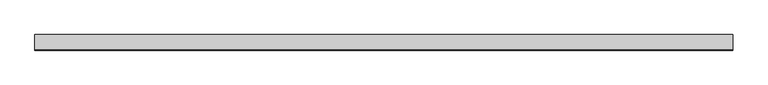
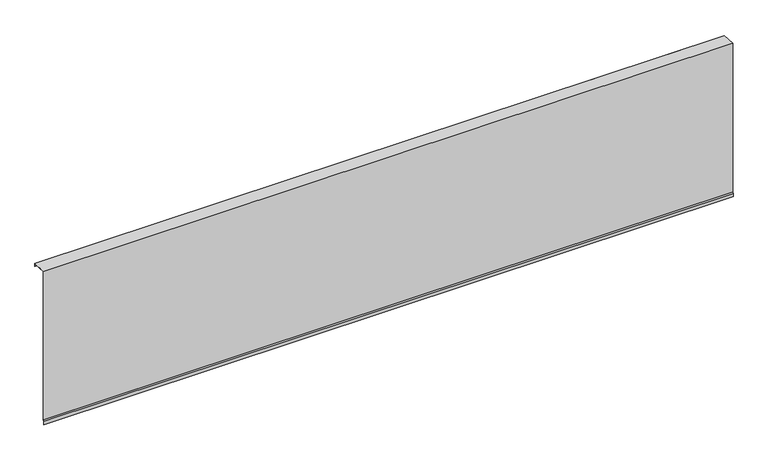
"""IFC4 building model written with IfcOpenShell, lengths in millimetres: proxy geometry, Generic Models 7:Generic Models 1:5:Generic Models 1:5 : Generic Models 7:Generic Models 1:337419:32 : Generic Models 7:Generic Models 1:5:Generic Models 1:5 : Generic Models 7:Generic Models 1:337419:311462."""

from ifc_helpers import new_model, si_unit, frame, origin, place, context, project, spatial, polyline, outline, extrude, source, transform, mapped, element, save


def generic_models_75d0ed6d(model_context):
    return source(origin(), model_context, "Body", "SweptSolid", [
        extrude(outline(polyline([(-579014.1851341, 3795.8885169), (-579025.7575229, 3779.361433), (-579025.7575229, 3725.3283058), (-579027.3450229, 3725.3283058), (-579027.3450229, 3779.8619698), (-579015.7726341, 3796.3890538), (-579015.7726341, 6180.6116872), (-578793.4990368, 6168.9628216), (-578793.4990368, 6125.115987), (-578795.0865368, 6125.115987), (-578795.0865368, 6167.4563403), (-579014.1851341, 6178.9388113), (-579014.1851341, 3795.8885169)])), frame((793360.8632437, 0.0, 0.0), z_axis=(1.0, 0.0, 0.0), x_axis=(0.0, 1.0, 0.0)), (0.0, 0.0, 1.0), 10452.1),
    ])


if __name__ == "__main__":
    model = new_model("IFC4")
    model_context = context("Model", 3, world=origin())
    ifc_project = project(units=[si_unit("LENGTHUNIT", "METRE", prefix="MILLI")], contexts=[model_context])
    site = spatial("IfcSite", under=ifc_project)
    building = spatial("IfcBuilding", under=site)
    placement = place(None, origin())
    generic_models_shape = generic_models_75d0ed6d(model_context)
    element("IfcBuildingElementProxy", 1, Name="Generic Models 7:Generic Models 1:5:Generic Models 1:5 : Generic Models 7:Generic Models 1:337419:32 : Generic Models 7:Generic Models 1:5:Generic Models 1:5 : Generic Models 7:Generic Models 1:337419:311462", ObjectType="Generic Models 7:Generic Models 1:5:Generic Models 1:5 : Generic Models 7:Generic Models 1:337419:32 : Generic Models 7:Generic Models 1:5:Generic Models 1:5 : Generic Models 7:Generic Models 1:337419:311462", at=placement, inside=building, context=model_context, shape_type="MappedRepresentation", body=[
        mapped(generic_models_shape, transform((0.0, 0.0, 0.0), x_axis=(1.0, 0.0, 0.0), y_axis=(0.0, 1.0, 0.0), z_axis=(0.0, 0.0, 1.0))),
    ])
    save(model, "model.ifc")

# Revit data of these elements
# Type "Generic Models 7:Generic Models 1:5:Generic Models 1:5 : Generic Models 7:Generic Models 1:337419:32 : Generic Models 7:Generic Models 1:5:Generic Models 1:5 : Generic Models 7:Generic Models 1:337419:311462"
#   NameOverride = "Generic Models 7:Generic Models 1:5:Generic Models 1:5 : Generic Models 7:Generic Models 1:337419:311462"
#   ObjectTypeOverride = "Generic Models 1:5 : Generic Models 7:Generic Models 1:337419"
#   Reference = "Generic Models 1"
#   Tag = "311462"
# Element 1 (IfcBuildingElementProxy, "Generic Models 7:Generic Models 1:5:Generic Models 1:5 : Generic Models 7:Generic Models 1:337419:32 : Generic Models 7:Generic Models 1:5:Generic Models 1:5 : Generic Models 7:Generic Models 1:337419:311462")
#   Materials on its faces: "UV STABLE WATER RESISTANT VAPOR PERMEABLE AIR BARRIER"
# Materials
#   "UV STABLE WATER RESISTANT VAPOR PERMEABLE AIR BARRIER": class "Generic", colour RGB 51 162 45, transparency 0, Description = "Polyethylene film membrane", Cost = 0
